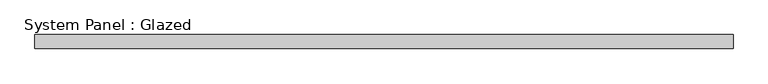
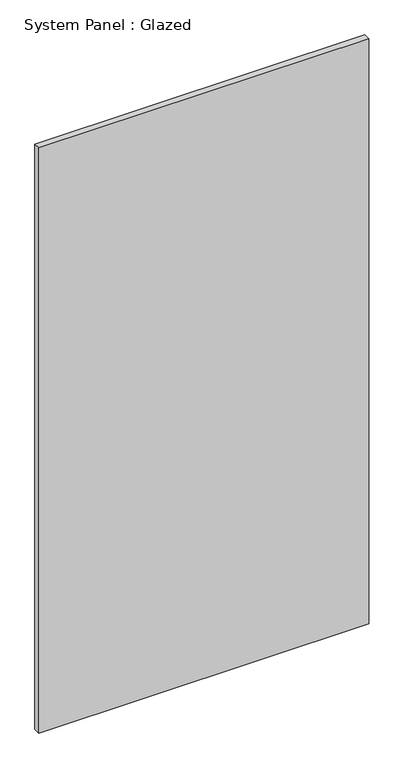
"""IFC4 building model written with IfcOpenShell, lengths in millimetres: plate geometry, System Panel : Glazed."""

from ifc_helpers import new_model, si_unit, origin, origin_with_axes, place, context, project, spatial, polyline, outline, extrude, source, transform, mapped, element, save


def system_panel_glazed_da598795(model_context):
    return source(origin(), model_context, "Body", "SweptSolid", [
        extrude(outline(polyline([(620.0000001, 24.5), (-620.0000001, 24.5), (-620.0000001, 49.5), (620.0000001, 49.5), (620.0000001, 24.5)])), origin_with_axes(), (0.0, 0.0, 1.0), 2325.0),
    ])


if __name__ == "__main__":
    model = new_model("IFC4")
    model_context = context("Model", 3, world=origin())
    ifc_project = project(units=[si_unit("LENGTHUNIT", "METRE", prefix="MILLI")], contexts=[model_context])
    site = spatial("IfcSite", under=ifc_project)
    building = spatial("IfcBuilding", under=site)
    placement = place(None, origin())
    system_panel_glazed_shape = system_panel_glazed_da598795(model_context)
    element("IfcPlate", 1, ObjectType="System Panel : Glazed", at=placement, inside=building, context=model_context, shape_type="MappedRepresentation", body=[
        mapped(system_panel_glazed_shape, transform((0.0, 0.0, 0.0), x_axis=(1.0, 0.0, 0.0), y_axis=(0.0, 1.0, 0.0), z_axis=(0.0, 0.0, 1.0))),
    ])
    save(model, "model.ifc")

# Revit data of these elements
# Type "System Panel : Glazed"
#   Construction Type Id = "GSP4R"
#   Analytic Construction = "1/8 in Pilkington single glazing"
#   Visual Light Transmittance = 0.9
#   Solar Heat Gain Coefficient = 0.86
#   Heat Transfer Coefficient (U) = 6.7069 W/(m²·K)
#   Define Thermal Properties by = 1
# Element 1 (IfcPlate, "System Panel : Glazed")
#   Materials on its faces: "Glass"
# Materials
#   "Glass": class "Glass", colour RGB 0 128 192, transparency 0.9, Description = "Soda Lime Glass", Cost = 0
